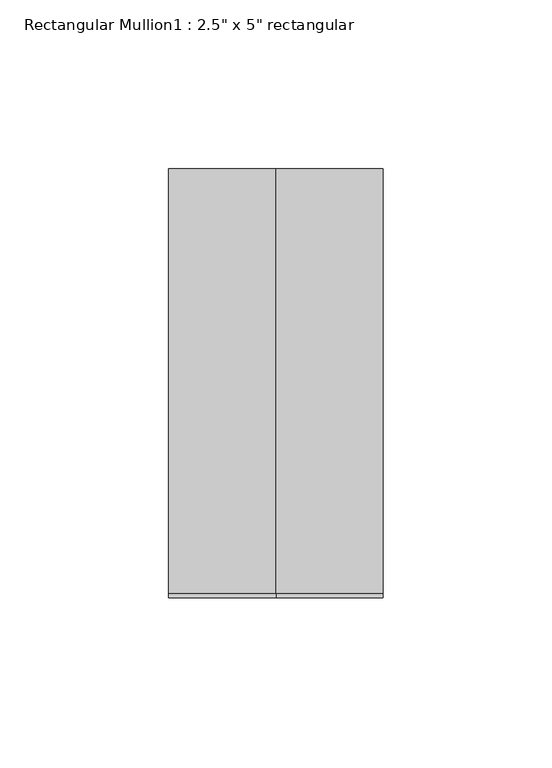
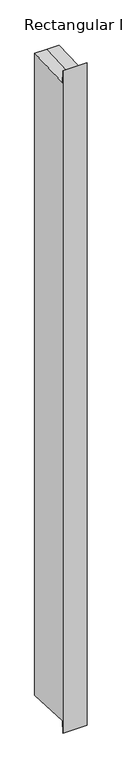
"""IFC4 building model written with IfcOpenShell, lengths in millimetres: member geometry."""

from ifc_helpers import new_model, si_unit, origin, place, context, project, spatial, faceted_brep, source, transform, mapped, element, save


def member_079229cb(model_context):
    return source(origin(), model_context, "Body", "Brep", [
        faceted_brep([(-31.75, 63.5, 2.5257955), (0.0, 63.5, 2.5257955), (31.75, 63.5, 2.5257955), (31.75, 63.5, -1767.8257955), (0.0, 63.5, -1767.8257955), (-31.75, 63.5, -1767.8257955), (-31.75, -63.5, 30.4748075), (-31.75, -62.174126, -2.5237591), (-31.75, -62.174126, -1762.7762409), (-31.75, -63.5, -1795.7748075), (31.75, -63.5, 30.4748075), (0.0, -63.5, 30.4748075), (0.0, -63.5, -1795.7748075), (31.75, -63.5, -1795.7748075), (31.75, -62.174126, -2.5237591), (31.75, -62.174126, -1762.7762409), (0.0, -62.174126, -2.5237591), (0.0, -62.174126, -1762.7762409)], [[[0, 1, 2, 3, 4, 5]], [[6, 7, 0, 5, 8, 9]], [[10, 11, 6, 9, 12, 13]], [[2, 14, 10, 13, 15, 3]], [[2, 1, 16, 14]], [[1, 0, 7, 16]], [[7, 6, 11, 16]], [[11, 10, 14, 16]], [[3, 15, 17, 4]], [[15, 13, 12, 17]], [[12, 9, 8, 17]], [[8, 5, 4, 17]]]),
    ])


if __name__ == "__main__":
    model = new_model("IFC4")
    model_context = context("Model", 3, world=origin())
    ifc_project = project(units=[si_unit("LENGTHUNIT", "METRE", prefix="MILLI")], contexts=[model_context])
    site = spatial("IfcSite", under=ifc_project)
    building = spatial("IfcBuilding", under=site)
    placement = place(None, origin())
    member_shape = member_079229cb(model_context)
    element("IfcMember", 1, ObjectType="Rectangular Mullion1 : 2.5\" x 5\" rectangular", at=placement, inside=building, context=model_context, shape_type="MappedRepresentation", body=[
        mapped(member_shape, transform((0.0, 0.0, 0.0), x_axis=(1.0, 0.0, 0.0), y_axis=(0.0, 1.0, 0.0), z_axis=(0.0, 0.0, 1.0))),
    ])
    save(model, "model.ifc")

# Revit data of these elements
# Type "Rectangular Mullion1 : 2.5\" x 5\" rectangular"
#   built-in parameter 1007304 = 0.416667 (stored number, unit not read)
#   built-in parameter 1007301 = 0.104167 (stored number, unit not read)
#   built-in parameter 1007300 = 0.104167 (stored number, unit not read)
# Element 1 (IfcMember, "Rectangular Mullion1 : 2.5\" x 5\" rectangular")
#   Materials on its faces: "support-frame"
# Materials
#   "support-frame": class "Unassigned", colour RGB 233 233 233, transparency 0, Cost = 0
